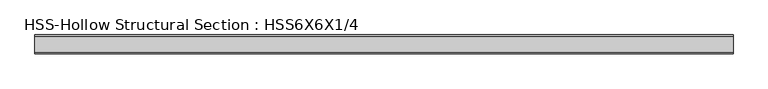
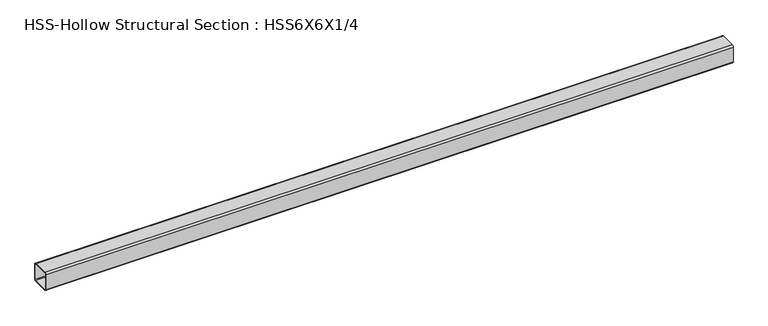
"""IFC4 building model written with IfcOpenShell, lengths in millimetres: beam geometry, HSS-Hollow Structural Section : HSS6X6X1/4."""

from ifc_helpers import new_model, si_unit, point, frame, frame_2d, origin, place, context, project, spatial, polyline, circle_curve, trimmed, segment, composite_curve, outline, extrude, source, transform, mapped, element, save


def hss_hollow_structural_section_hss6x6x1_4_4ad22346(model_context):
    return source(origin(), model_context, "Body", "SweptSolid", [
        extrude(outline(composite_curve([segment(polyline([(76.2, 64.3636), (76.2, -64.3636)]), True, "CONTINUOUS"), segment(trimmed(circle_curve(frame_2d((64.3636, -64.3636)), 11.8364), [point((76.2, -64.3636))], [point((64.3636, -76.2))], False, "CARTESIAN"), True, "CONTINUOUS"), segment(polyline([(64.3636, -76.2), (-64.3636, -76.2)]), True, "CONTINUOUS"), segment(trimmed(circle_curve(frame_2d((-64.3636, -64.3636)), 11.8364), [point((-64.3636, -76.2))], [point((-76.2, -64.3636))], False, "CARTESIAN"), True, "CONTINUOUS"), segment(polyline([(-76.2, -64.3636), (-76.2, 64.3636)]), True, "CONTINUOUS"), segment(trimmed(circle_curve(frame_2d((-64.3636, 64.3636)), 11.8364), [point((-76.2, 64.3636))], [point((-64.3636, 76.2))], False, "CARTESIAN"), True, "CONTINUOUS"), segment(polyline([(-64.3636, 76.2), (64.3636, 76.2)]), True, "CONTINUOUS"), segment(trimmed(circle_curve(frame_2d((64.3636, 64.3636)), 11.8364), [point((64.3636, 76.2))], [point((76.2, 64.3636))], False, "CARTESIAN"), True, "CONTINUOUS")], self_intersect=False), holes=[composite_curve([segment(trimmed(circle_curve(frame_2d((-64.3636, 64.3636)), 5.9182), [point((-64.3636, 70.2818))], [point((-70.2818, 64.3636))], True, "CARTESIAN"), True, "CONTINUOUS"), segment(polyline([(-70.2818, 64.3636), (-70.2818, -64.3636)]), True, "CONTINUOUS"), segment(trimmed(circle_curve(frame_2d((-64.3636, -64.3636)), 5.9182), [point((-70.2818, -64.3636))], [point((-64.3636, -70.2818))], True, "CARTESIAN"), True, "CONTINUOUS"), segment(polyline([(-64.3636, -70.2818), (64.3636, -70.2818)]), True, "CONTINUOUS"), segment(trimmed(circle_curve(frame_2d((64.3636, -64.3636)), 5.9182), [point((64.3636, -70.2818))], [point((70.2818, -64.3636))], True, "CARTESIAN"), True, "CONTINUOUS"), segment(polyline([(70.2818, -64.3636), (70.2818, 64.3636)]), True, "CONTINUOUS"), segment(trimmed(circle_curve(frame_2d((64.3636, 64.3636)), 5.9182), [point((70.2818, 64.3636))], [point((64.3636, 70.2818))], True, "CARTESIAN"), True, "CONTINUOUS"), segment(polyline([(64.3636, 70.2818), (-64.3636, 70.2818)]), True, "CONTINUOUS")], self_intersect=False)]), frame((-2844.8, 0.0, 0.0), z_axis=(1.0, 0.0, 0.0), x_axis=(0.0, 1.0, 0.0)), (0.0, 0.0, 1.0), 5600.7),
    ])


if __name__ == "__main__":
    model = new_model("IFC4")
    model_context = context("Model", 3, world=origin())
    ifc_project = project(units=[si_unit("LENGTHUNIT", "METRE", prefix="MILLI")], contexts=[model_context])
    site = spatial("IfcSite", under=ifc_project)
    building = spatial("IfcBuilding", under=site)
    placement = place(None, origin())
    hss_hollow_structural_section_hss6x6x1_4_shape = hss_hollow_structural_section_hss6x6x1_4_4ad22346(model_context)
    element("IfcBeam", 1, ObjectType="HSS-Hollow Structural Section : HSS6X6X1/4", at=placement, inside=building, context=model_context, shape_type="MappedRepresentation", body=[
        mapped(hss_hollow_structural_section_hss6x6x1_4_shape, transform((0.0, 0.0, 0.0), x_axis=(1.0, 0.0, 0.0), y_axis=(0.0, 1.0, 0.0), z_axis=(0.0, 0.0, 1.0))),
    ])
    save(model, "model.ifc")

# Revit data of these elements
# Type "HSS-Hollow Structural Section : HSS6X6X1/4"
#   Assembly Code = "B10"
#   Shape = "Square"
#   W = 19
#   Ht = 0' - 6"
#   Length [instance default] = 5' - 0"
#   b = 0' - 6"
#   kr = 0' - 0.466"
#   t = 0' - 0.233"
#   A = 0.0363889 SF
#   Structural Material [instance default] = Steel ASTM A500, Grade B, Rectangular and Square
# Element 1 (IfcBeam, "HSS-Hollow Structural Section : HSS6X6X1/4")
#   Materials on its faces: "Steel ASTM A500, Grade B, Rectangular and Square"
# Materials
#   "Steel ASTM A500, Grade B, Rectangular and Square": class "Metal", colour RGB 199 199 199, transparency 0, Description = "Carbon steel", Cost = 0
